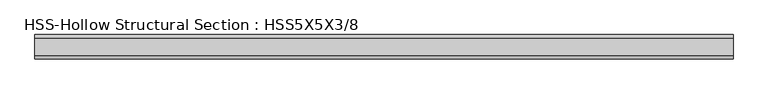
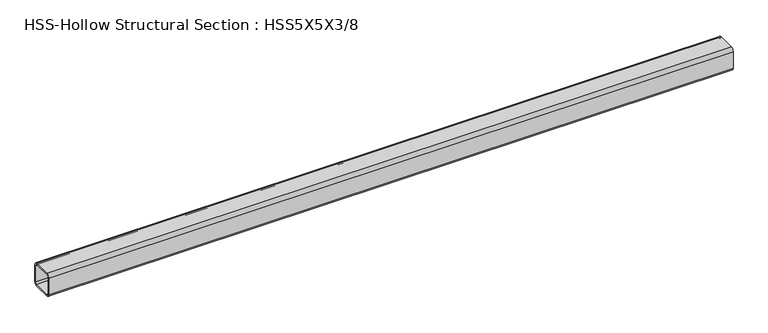
"""IFC4 building model written with IfcOpenShell, lengths in millimetres: beam geometry, HSS-Hollow Structural Section : HSS5X5X3/8."""

import ifcopenshell
import ifcopenshell.guid

model = None  # the IFC model being written
_history = None  # IfcOwnerHistory: only IFC2X3 demands one
_inside = {}  # id of a spatial element -> (the spatial element, [elements in it])
_under = {}  # id of a project, library or spatial element -> (it, [spatial elements below it])
_declared = {}  # id of a project -> (the project, [libraries it declares])
_typed = {}  # id of a type object -> (the type object, [elements of that type])
_made_of = {}  # id of a material, layer set ... -> (it, [elements and type objects made of it])


def new_model(schema):
    """Start an empty IFC model of exactly this schema.

    Asked for "IFC4X3", IfcOpenShell would pick the latest addendum, in which some entities
    have other attributes; the version numbers below select the first issue.
    IFC2X3 requires an IfcOwnerHistory on every rooted entity: one is made here for all.
    """
    global model, _history
    if schema == "IFC4X3":
        model = ifcopenshell.file(schema_version=(4, 3, 0, 0))
    else:
        model = ifcopenshell.file(schema=schema)
    _inside.clear()
    _under.clear()
    _declared.clear()
    _typed.clear()
    _made_of.clear()
    _history = None
    if model.schema == "IFC2X3":
        org = make("IfcOrganization", Name="unknown")
        user = make(
            "IfcPersonAndOrganization",
            ThePerson=make("IfcPerson", FamilyName="unknown"),
            TheOrganization=org,
        )
        app = make(
            "IfcApplication",
            ApplicationDeveloper=org,
            Version="unknown",
            ApplicationFullName="unknown",
            ApplicationIdentifier="unknown",
        )
        _history = make(
            "IfcOwnerHistory",
            OwningUser=user,
            OwningApplication=app,
            ChangeAction="ADDED",
            CreationDate=0,
        )
    return model


def make(cls, **values):
    """One entity of the class cls with the attributes given. An attribute that is None is left unset."""
    return model.create_entity(
        cls, **{name: value for name, value in values.items() if value is not None}
    )


def rooted(cls, **values):
    """An entity with a GlobalId (a new one), such as an element, a storey or a relation."""
    return make(cls, GlobalId=ifcopenshell.guid.new(), OwnerHistory=_history, **values)


def si_unit(unit_type, name, prefix=None):
    """IfcSIUnit, for example si_unit("LENGTHUNIT", "METRE", prefix="MILLI")."""
    return make("IfcSIUnit", UnitType=unit_type, Prefix=prefix, Name=name)


def assignment(units):
    """IfcUnitAssignment: the units of a project."""
    return None if units is None else make("IfcUnitAssignment", Units=units)


def point(xyz):
    """IfcCartesianPoint."""
    return None if xyz is None else make("IfcCartesianPoint", Coordinates=xyz)


def direction(xyz):
    """IfcDirection."""
    return None if xyz is None else make("IfcDirection", DirectionRatios=xyz)


def frame(location, z_axis=None, x_axis=None):
    """IfcAxis2Placement3D, a coordinate frame: its origin and axes. An axis left out is left unset."""
    return make(
        "IfcAxis2Placement3D",
        Location=point(location),
        Axis=direction(z_axis),
        RefDirection=direction(x_axis),
    )


def frame_2d(location, x_axis=None):
    """IfcAxis2Placement2D, a coordinate frame in the plane: its origin and x axis."""
    return make(
        "IfcAxis2Placement2D", Location=point(location), RefDirection=direction(x_axis)
    )


def origin():
    """The frame at (0, 0, 0) with its axes left unset."""
    return frame((0.0, 0.0, 0.0))


def place(relative_to, where):
    """IfcLocalPlacement: puts the frame where relative to a parent placement (None: the world)."""
    return make(
        "IfcLocalPlacement", PlacementRelTo=relative_to, RelativePlacement=where
    )


def context(
    kind, dimensions, precision=None, world=None, true_north=None, identifier=None
):
    """IfcGeometricRepresentationContext, for example the 3D "Model" context."""
    return make(
        "IfcGeometricRepresentationContext",
        ContextIdentifier=identifier,
        ContextType=kind,
        CoordinateSpaceDimension=dimensions,
        Precision=precision,
        WorldCoordinateSystem=world,
        TrueNorth=true_north,
    )


def project(units=None, contexts=None):
    """IfcProject with its units and contexts."""
    return rooted(
        "IfcProject",
        Name="project",
        RepresentationContexts=contexts,
        UnitsInContext=assignment(units),
    )


def spatial(cls, under=None, at=None, **own):
    """A site, building, storey or space (cls), placed at a placement, below another one or the project."""
    s = rooted(cls, ObjectPlacement=at, **own)
    if under is not None:
        _under.setdefault(under.id(), (under, []))[1].append(s)
    return s


def polyline(points):
    """IfcPolyline through the points."""
    return make("IfcPolyline", Points=[point(p) for p in points])


def circle_curve(where, radius):
    """IfcCircle in the frame where."""
    return make("IfcCircle", Position=where, Radius=radius)


def trimmed(basis, trim1, trim2, sense, master):
    """IfcTrimmedCurve: the piece of a basis curve between two trims."""
    return make(
        "IfcTrimmedCurve",
        BasisCurve=basis,
        Trim1=trim1,
        Trim2=trim2,
        SenseAgreement=sense,
        MasterRepresentation=master,
    )


def segment(curve, same_sense, transition):
    """IfcCompositeCurveSegment."""
    return make(
        "IfcCompositeCurveSegment",
        Transition=transition,
        SameSense=same_sense,
        ParentCurve=curve,
    )


def composite_curve(segments, self_intersect=None):
    """IfcCompositeCurve: segments joined end to end."""
    return make("IfcCompositeCurve", Segments=segments, SelfIntersect=self_intersect)


def outline(outer, holes=None, kind="AREA"):
    """IfcArbitraryClosedProfileDef: a profile drawn as a closed curve; with holes, ...WithVoids."""
    if holes is None:
        return make("IfcArbitraryClosedProfileDef", ProfileType=kind, OuterCurve=outer)
    return make(
        "IfcArbitraryProfileDefWithVoids",
        ProfileType=kind,
        OuterCurve=outer,
        InnerCurves=holes,
    )


def extrude(swept, where, along, depth):
    """IfcExtrudedAreaSolid: the profile swept, set in the frame where, extruded along a direction by depth."""
    return make(
        "IfcExtrudedAreaSolid",
        SweptArea=swept,
        Position=where,
        ExtrudedDirection=direction(along),
        Depth=depth,
    )


def shape(context_of_items, identifier, shape_type, items):
    """IfcShapeRepresentation: the items that make up one representation, for example the "Body"."""
    return make(
        "IfcShapeRepresentation",
        ContextOfItems=context_of_items,
        RepresentationIdentifier=identifier,
        RepresentationType=shape_type,
        Items=items,
    )


def source(mapping_origin, context_of_items, identifier, shape_type, items):
    """IfcRepresentationMap: a shape defined once, which mapped items show again and again."""
    return make(
        "IfcRepresentationMap",
        MappingOrigin=mapping_origin,
        MappedRepresentation=shape(context_of_items, identifier, shape_type, items),
    )


def transform(
    local_origin,
    x_axis=None,
    y_axis=None,
    z_axis=None,
    scale=None,
    scale2=None,
    scale3=None,
    uniform=True,
):
    """IfcCartesianTransformationOperator3D, or its non-uniform kind. x_axis, y_axis, z_axis: its Axis1, 2, 3."""
    if uniform:
        return make(
            "IfcCartesianTransformationOperator3D",
            Axis1=direction(x_axis),
            Axis2=direction(y_axis),
            LocalOrigin=point(local_origin),
            Scale=scale,
            Axis3=direction(z_axis),
        )
    return make(
        "IfcCartesianTransformationOperator3DnonUniform",
        Axis1=direction(x_axis),
        Axis2=direction(y_axis),
        LocalOrigin=point(local_origin),
        Scale=scale,
        Axis3=direction(z_axis),
        Scale2=scale2,
        Scale3=scale3,
    )


def mapped(mapping_source, mapping_target):
    """IfcMappedItem: shows the shape of a source again, moved by a transform."""
    return make(
        "IfcMappedItem", MappingSource=mapping_source, MappingTarget=mapping_target
    )


def made_of(thing, what):
    """Note that an element or type object is made of a material, layer set ...; save() writes the relation."""
    if what is not None:
        _made_of.setdefault(what.id(), (what, []))[1].append(thing)
    return thing


def element(
    cls,
    number,
    at=None,
    inside=None,
    cuts=None,
    type_object=None,
    material=None,
    context=None,
    identifier="Body",
    shape_type=None,
    held_by="IfcProductDefinitionShape",
    body=None,
    shapes=None,
    **own,
):
    """One element of the class cls, such as IfcWall. Its Tag is "e" and its number.

    at: its placement. inside: the storey or other place that contains it. cuts: it is an
    opening in that element (IfcRelVoidsElement). A single representation is given by context,
    identifier, shape_type and body (its items); several are given by shapes. held_by: the class
    of the entity that holds the representations. save() writes the other relations.
    """
    e = rooted(cls, Tag="e%d" % number, ObjectPlacement=at, **own)
    if body is not None:
        shapes = [shape(context, identifier, shape_type, body)]
    if shapes is not None:
        e.Representation = make(held_by, Representations=shapes)
    if inside is not None:
        _inside.setdefault(inside.id(), (inside, []))[1].append(e)
    if cuts is not None:
        rooted(
            "IfcRelVoidsElement", RelatingBuildingElement=cuts, RelatedOpeningElement=e
        )
    if type_object is not None:
        _typed.setdefault(type_object.id(), (type_object, []))[1].append(e)
    return made_of(e, material)


def aggregate(whole, parts):
    """IfcRelAggregates: a whole, such as a stair, and the parts it consists of."""
    return rooted("IfcRelAggregates", RelatingObject=whole, RelatedObjects=parts)


def save(model, path):
    """Write the relations noted so far, then the file.

    IfcRelAggregates (storeys below a building ...), IfcRelContainedInSpatialStructure (elements
    in a storey), IfcRelDefinesByType, IfcRelAssociatesMaterial and IfcRelDeclares: one each for
    every whole, place, type object, material and project.
    """
    for whole, parts in _under.values():
        aggregate(whole, parts)
    for where, things in _inside.values():
        rooted(
            "IfcRelContainedInSpatialStructure",
            RelatedElements=things,
            RelatingStructure=where,
        )
    for kind, things in _typed.values():
        rooted("IfcRelDefinesByType", RelatedObjects=things, RelatingType=kind)
    for what, things in _made_of.values():
        rooted("IfcRelAssociatesMaterial", RelatedObjects=things, RelatingMaterial=what)
    for by, libraries in _declared.values():
        rooted("IfcRelDeclares", RelatingContext=by, RelatedDefinitions=libraries)
    model.write(path)


def hss_hollow_structural_section_hss5x5x3_8_b32892de(model_context):
    return source(origin(), model_context, "Body", "SweptSolid", [
        extrude(outline(composite_curve([segment(polyline([(63.5, 45.7708), (63.5, -45.7708)]), True, "CONTINUOUS"), segment(trimmed(circle_curve(frame_2d((45.7708, -45.7708)), 17.7292), [point((63.5, -45.7708))], [point((45.7708, -63.5))], False, "CARTESIAN"), True, "CONTINUOUS"), segment(polyline([(45.7708, -63.5), (-45.7708, -63.5)]), True, "CONTINUOUS"), segment(trimmed(circle_curve(frame_2d((-45.7708, -45.7708)), 17.7292), [point((-45.7708, -63.5))], [point((-63.5, -45.7708))], False, "CARTESIAN"), True, "CONTINUOUS"), segment(polyline([(-63.5, -45.7708), (-63.5, 45.7708)]), True, "CONTINUOUS"), segment(trimmed(circle_curve(frame_2d((-45.7708, 45.7708)), 17.7292), [point((-63.5, 45.7708))], [point((-45.7708, 63.5))], False, "CARTESIAN"), True, "CONTINUOUS"), segment(polyline([(-45.7708, 63.5), (45.7708, 63.5)]), True, "CONTINUOUS"), segment(trimmed(circle_curve(frame_2d((45.7708, 45.7708)), 17.7292), [point((45.7708, 63.5))], [point((63.5, 45.7708))], False, "CARTESIAN"), True, "CONTINUOUS")], self_intersect=False), holes=[composite_curve([segment(trimmed(circle_curve(frame_2d((-45.7708, 45.7708)), 8.8646), [point((-45.7708, 54.6354))], [point((-54.6354, 45.7708))], True, "CARTESIAN"), True, "CONTINUOUS"), segment(polyline([(-54.6354, 45.7708), (-54.6354, -45.7708)]), True, "CONTINUOUS"), segment(trimmed(circle_curve(frame_2d((-45.7708, -45.7708)), 8.8646), [point((-54.6354, -45.7708))], [point((-45.7708, -54.6354))], True, "CARTESIAN"), True, "CONTINUOUS"), segment(polyline([(-45.7708, -54.6354), (45.7708, -54.6354)]), True, "CONTINUOUS"), segment(trimmed(circle_curve(frame_2d((45.7708, -45.7708)), 8.8646), [point((45.7708, -54.6354))], [point((54.6354, -45.7708))], True, "CARTESIAN"), True, "CONTINUOUS"), segment(polyline([(54.6354, -45.7708), (54.6354, 45.7708)]), True, "CONTINUOUS"), segment(trimmed(circle_curve(frame_2d((45.7708, 45.7708)), 8.8646), [point((54.6354, 45.7708))], [point((45.7708, 54.6354))], True, "CARTESIAN"), True, "CONTINUOUS"), segment(polyline([(45.7708, 54.6354), (-45.7708, 54.6354)]), True, "CONTINUOUS")], self_intersect=False)]), frame((-1819.275, 0.0, 0.0), z_axis=(1.0, 0.0, 0.0), x_axis=(0.0, 1.0, 0.0)), (0.0, 0.0, 1.0), 3638.55),
    ])


if __name__ == "__main__":
    model = new_model("IFC4")
    model_context = context("Model", 3, world=origin())
    ifc_project = project(units=[si_unit("LENGTHUNIT", "METRE", prefix="MILLI")], contexts=[model_context])
    site = spatial("IfcSite", under=ifc_project)
    building = spatial("IfcBuilding", under=site)
    placement = place(None, origin())
    hss_hollow_structural_section_hss5x5x3_8_shape = hss_hollow_structural_section_hss5x5x3_8_b32892de(model_context)
    element("IfcBeam", 1, ObjectType="HSS-Hollow Structural Section : HSS5X5X3/8", at=placement, inside=building, context=model_context, shape_type="MappedRepresentation", body=[
        mapped(hss_hollow_structural_section_hss5x5x3_8_shape, transform((0.0, 0.0, 0.0), x_axis=(1.0, 0.0, 0.0), y_axis=(0.0, 1.0, 0.0), z_axis=(0.0, 0.0, 1.0))),
    ])
    save(model, "model.ifc")

# Revit data of these elements
# Type "HSS-Hollow Structural Section : HSS5X5X3/8"
#   Assembly Code = "B10"
#   Shape = "Square"
#   W = 22.3
#   Ht = 0' - 5"
#   Length [instance default] = 5' - 0"
#   b = 0' - 5"
#   kr = 0' - 0.698"
#   t = 0' - 0.349"
#   A = 0.0429167 SF
#   Structural Material [instance default] = Steel ASTM A500, Grade B, Rectangular and Square
# Element 1 (IfcBeam, "HSS-Hollow Structural Section : HSS5X5X3/8")
#   Materials on its faces: "Steel ASTM A500, Grade B, Rectangular and Square"
# Materials
#   "Steel ASTM A500, Grade B, Rectangular and Square": class "Metal", colour RGB 199 199 199, transparency 0, Description = "Carbon steel", Cost = 0
